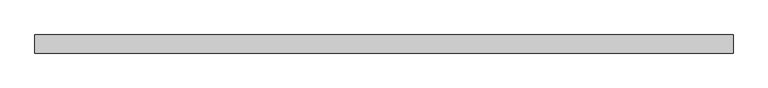
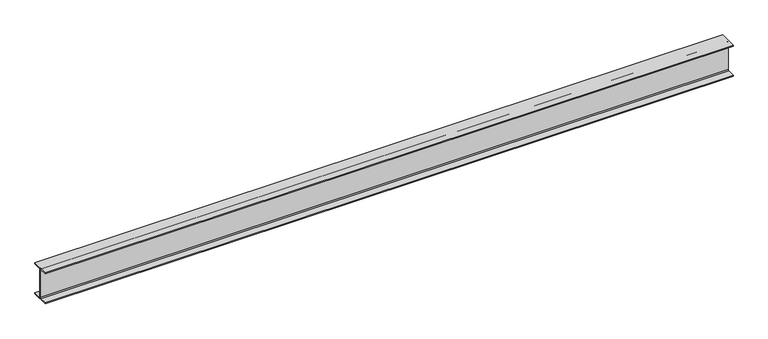
"""IFC4 building model written with IfcOpenShell, lengths in millimetres: beam geometry, Old_Steel Beam_H-KSD3502 : H_SB_ASB_H-390×300x10x16."""

from ifc_helpers import new_model, si_unit, point, frame, frame_2d, origin, place, context, project, spatial, polyline, circle_curve, trimmed, segment, composite_curve, outline, extrude, source, transform, mapped, element, save


def beam_5c6733fe(model_context):
    return source(origin(), model_context, "Body", "SweptSolid", [
        extrude(outline(composite_curve([segment(polyline([(82.5, -141.5), (82.5, -151.7), (-82.5, -151.7), (-82.5, -141.5), (-11.9, -141.5)]), True, "CONTINUOUS"), segment(trimmed(circle_curve(frame_2d((-11.9, -132.6)), 8.9), [point((-11.9, -141.5))], [point((-3.0, -132.6))], True, "CARTESIAN"), True, "CONTINUOUS"), segment(polyline([(-3.0, -132.6), (-3.0, 132.6)]), True, "CONTINUOUS"), segment(trimmed(circle_curve(frame_2d((-11.9, 132.6)), 8.9), [point((-3.0, 132.6))], [point((-11.9, 141.5))], True, "CARTESIAN"), True, "CONTINUOUS"), segment(polyline([(-11.9, 141.5), (-82.5, 141.5), (-82.5, 151.7), (82.5, 151.7), (82.5, 141.5), (11.9, 141.5)]), True, "CONTINUOUS"), segment(trimmed(circle_curve(frame_2d((11.9, 132.6)), 8.9), [point((11.9, 141.5))], [point((3.0, 132.6))], True, "CARTESIAN"), True, "CONTINUOUS"), segment(polyline([(3.0, 132.6), (3.0, -132.6)]), True, "CONTINUOUS"), segment(trimmed(circle_curve(frame_2d((11.9, -132.6)), 8.9), [point((3.0, -132.6))], [point((11.9, -141.5))], True, "CARTESIAN"), True, "CONTINUOUS"), segment(polyline([(11.9, -141.5), (82.5, -141.5)]), True, "CONTINUOUS")], self_intersect=False)), frame((-2987.2999994, 0.0, 0.0), z_axis=(1.0, 0.0, 0.0), x_axis=(0.0, 1.0, 0.0)), (0.0, 0.0, 1.0), 6366.9040188),
    ])


if __name__ == "__main__":
    model = new_model("IFC4")
    model_context = context("Model", 3, world=origin())
    ifc_project = project(units=[si_unit("LENGTHUNIT", "METRE", prefix="MILLI")], contexts=[model_context])
    site = spatial("IfcSite", under=ifc_project)
    building = spatial("IfcBuilding", under=site)
    placement = place(None, origin())
    beam_shape = beam_5c6733fe(model_context)
    element("IfcBeam", 1, ObjectType="Old_Steel Beam_H-KSD3502 : H_SB_ASB_H-390×300x10x16", at=placement, inside=building, context=model_context, shape_type="MappedRepresentation", body=[
        mapped(beam_shape, transform((0.0, 0.0, 0.0), x_axis=(1.0, 0.0, 0.0), y_axis=(0.0, 1.0, 0.0), z_axis=(0.0, 0.0, 1.0))),
    ])
    save(model, "model.ifc")

# Revit data of these elements
# Type "Old_Steel Beam_H-KSD3502 : H_SB_ASB_H-390×300x10x16"
#   Width = 30.0 cm
#   Web Thickness = 1.0 cm
#   Web Fillet = 2.2 cm
#   Warping Constant = 2517770.0 cm⁶
#   Torsional Moment of Inertia = 94.3867 cm⁴
#   Torsional Modulus = 1.0 cm³
#   Section Area = 136.0 cm²
#   Plastic Modulus weak axis = 733.0 cm³
#   Plastic Modulus strong axis = 2190.0 cm³
#   Perimeter = 1.92 m²/m
#   Nominal Weight = 107.00 kgf/m
#   Moment of Inertia weak axis = 7210.00 cm⁴
#   Moment of Inertia strong axis = 38700.00 cm⁴
#   Height = 39.0 cm
#   Flange Thickness = 1.6 cm
#   Elastic Modulus weak axis = 481.0 cm³
#   Elastic Modulus strong axis = 1980.0 cm³
#   Centroid Vertical = 19.5 cm
#   Centroid Horizontal = 15.0 cm
#   Length [instance default] = 1.5240 m
#   Structural Material [instance default] = Steel, 45-345
#   Assembly Code = ""
# Element 1 (IfcBeam, "Old_Steel Beam_H-KSD3502 : H_SB_ASB_H-390×300x10x16")
#   Structural Material = none
# Materials
#   "Steel, 45-345": class "Metal", colour RGB 189 187 185, transparency 0, Description = "Steel 345 MPa", Cost = 0
